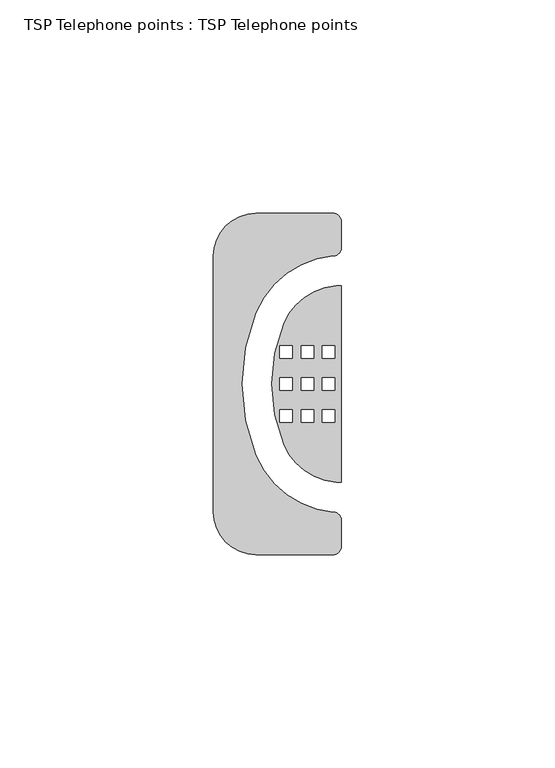
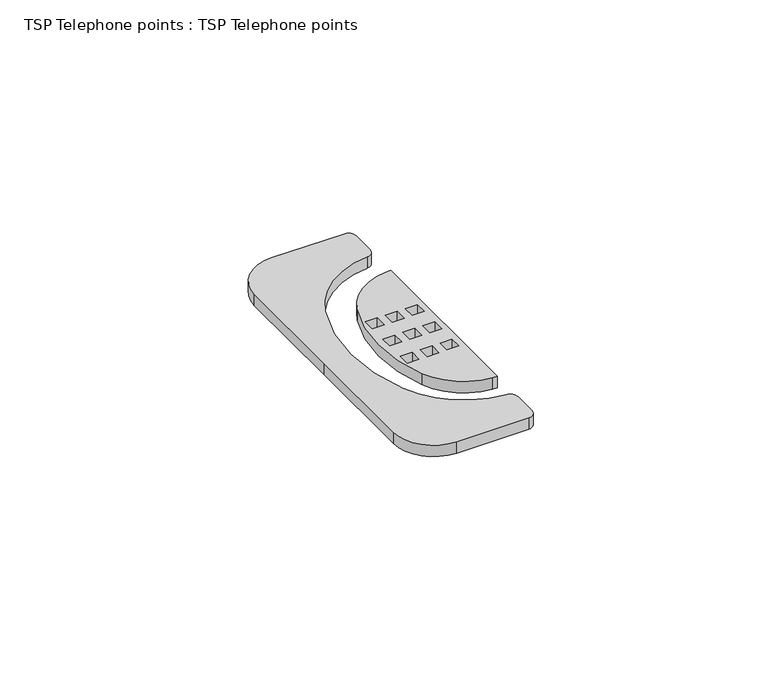
"""IFC4 building model written with IfcOpenShell, lengths in millimetres: proxy geometry, TSP Telephone points : TSP Telephone points."""

from ifc_helpers import new_model, si_unit, point, frame_2d, origin, origin_with_axes, place, context, project, spatial, polyline, circle_curve, trimmed, segment, composite_curve, outline, extrude, source, transform, mapped, element, save


def tsp_telephone_points_tsp_telephone_points_97399d21(model_context):
    return source(origin(), model_context, "Body", "SweptSolid", [
        extrude(outline(composite_curve([segment(polyline([(0.0, 38.0), (0.0, 32.0)]), True, "CONTINUOUS"), segment(trimmed(circle_curve(frame_2d((-2.0, 32.0)), 2.0), [point((0.0, 32.0))], [point((-1.8374907, 30.0066133))], False, "CARTESIAN"), True, "CONTINUOUS"), segment(trimmed(circle_curve(frame_2d((0.0, 8.4180035)), 21.6666667), [point((-1.8374907, 30.0066133))], [point((-20.0, 16.7513368))], True, "CARTESIAN"), True, "CONTINUOUS"), segment(trimmed(circle_curve(frame_2d((20.2032083, 0.0)), 43.5534757), [point((-20.0, 16.7513368))], [point((-20.0, -16.7513368))], True, "CARTESIAN"), True, "CONTINUOUS"), segment(trimmed(circle_curve(frame_2d((0.0, -8.4180035)), 21.6666667), [point((-20.0, -16.7513368))], [point((-1.8374907, -30.0066133))], True, "CARTESIAN"), True, "CONTINUOUS"), segment(trimmed(circle_curve(frame_2d((-2.0, -32.0)), 2.0), [point((-1.8374907, -30.0066133))], [point((0.0, -32.0))], False, "CARTESIAN"), True, "CONTINUOUS"), segment(polyline([(0.0, -32.0), (0.0, -38.0)]), True, "CONTINUOUS"), segment(trimmed(circle_curve(frame_2d((-2.0, -38.0)), 2.0), [point((0.0, -38.0))], [point((-2.0, -40.0))], False, "CARTESIAN"), True, "CONTINUOUS"), segment(polyline([(-2.0, -40.0), (-20.0, -40.0)]), True, "CONTINUOUS"), segment(trimmed(circle_curve(frame_2d((-20.0, -30.0)), 10.0), [point((-20.0, -40.0))], [point((-30.0, -30.0))], False, "CARTESIAN"), True, "CONTINUOUS"), segment(polyline([(-30.0, -30.0), (-30.0, 0.0), (-30.0, 30.0)]), True, "CONTINUOUS"), segment(trimmed(circle_curve(frame_2d((-20.0, 30.0)), 10.0), [point((-30.0, 30.0))], [point((-20.0, 40.0))], False, "CARTESIAN"), True, "CONTINUOUS"), segment(polyline([(-20.0, 40.0), (-2.0, 40.0)]), True, "CONTINUOUS"), segment(trimmed(circle_curve(frame_2d((-2.0, 38.0)), 2.0), [point((-2.0, 40.0))], [point((0.0, 38.0))], False, "CARTESIAN"), True, "CONTINUOUS")], self_intersect=False)), origin_with_axes(), (0.0, 0.0, 1.0), 3.0),
        extrude(outline(composite_curve([segment(trimmed(circle_curve(frame_2d((20.2032083, 0.0)), 36.5534757), [point((-13.5384615, -14.0590291))], [point((-13.5384615, 14.0590291))], False, "CARTESIAN"), True, "CONTINUOUS"), segment(trimmed(circle_curve(frame_2d((0.0, 8.4180035)), 14.6666667), [point((-13.5384615, 14.0590291))], [point((-1.2438398, 23.0318316))], False, "CARTESIAN"), True, "CONTINUOUS"), segment(polyline([(-1.2438398, 23.0318316), (0.0, 23.0318316), (0.0, -23.0318316), (-1.2438398, -23.0318316)]), True, "CONTINUOUS"), segment(trimmed(circle_curve(frame_2d((0.0, -8.4180035)), 14.6666667), [point((-1.2438398, -23.0318316))], [point((-13.5384615, -14.0590291))], False, "CARTESIAN"), True, "CONTINUOUS")], self_intersect=False), holes=[polyline([(-6.4751337, 9.0), (-9.4524255, 9.0), (-9.4524255, 6.0), (-6.4751337, 6.0), (-6.4751337, 9.0)]), polyline([(-11.4751337, 9.0), (-14.4524255, 9.0), (-14.4524255, 6.0), (-11.4751337, 6.0), (-11.4751337, 9.0)]), polyline([(-4.4751337, 9.0), (-4.4751337, 6.0), (-1.4978419, 6.0), (-1.4978419, 9.0), (-4.4751337, 9.0)]), polyline([(-6.4751337, -9.0), (-6.4751337, -6.0), (-9.4524255, -6.0), (-9.4524255, -9.0), (-6.4751337, -9.0)]), polyline([(-11.4751337, -9.0), (-11.4751337, -6.0), (-14.4524255, -6.0), (-14.4524255, -9.0), (-11.4751337, -9.0)]), polyline([(-4.4751337, -9.0), (-1.4978419, -9.0), (-1.4978419, -6.0), (-4.4751337, -6.0), (-4.4751337, -9.0)]), polyline([(-6.4751337, -1.5), (-6.4751337, 1.5), (-9.4524255, 1.5), (-9.4524255, -1.5), (-6.4751337, -1.5)]), polyline([(-11.4751337, -1.5), (-11.4751337, 1.5), (-14.4524255, 1.5), (-14.4524255, -1.5), (-11.4751337, -1.5)]), polyline([(-4.4751337, -1.5), (-1.4978419, -1.5), (-1.4978419, 1.5), (-4.4751337, 1.5), (-4.4751337, -1.5)])]), origin_with_axes(), (0.0, 0.0, 1.0), 3.0),
    ])


if __name__ == "__main__":
    model = new_model("IFC4")
    model_context = context("Model", 3, world=origin())
    ifc_project = project(units=[si_unit("LENGTHUNIT", "METRE", prefix="MILLI")], contexts=[model_context])
    site = spatial("IfcSite", under=ifc_project)
    building = spatial("IfcBuilding", under=site)
    placement = place(None, origin())
    tsp_telephone_points_tsp_telephone_points_shape = tsp_telephone_points_tsp_telephone_points_97399d21(model_context)
    element("IfcBuildingElementProxy", 1, Name="TSP Telephone points : TSP Telephone points", ObjectType="TSP Telephone points : TSP Telephone points", at=placement, inside=building, context=model_context, shape_type="MappedRepresentation", body=[
        mapped(tsp_telephone_points_tsp_telephone_points_shape, transform((0.0, 0.0, 0.0), x_axis=(1.0, 0.0, 0.0), y_axis=(0.0, 1.0, 0.0), z_axis=(0.0, 0.0, 1.0))),
    ])
    save(model, "model.ifc")

# Revit data of these elements
# Type "TSP Telephone points : TSP Telephone points"
#   Model = "TSP_ELECTELP"
#   Default Elevation = 0
# Element 1 (IfcBuildingElementProxy, "TSP Telephone points : TSP Telephone points")
#   Materials on its faces: "Cellulose Fill"
# Materials
#   "Cellulose Fill": class "Generic", colour RGB 0 0 0, transparency 0, Description = "Cellulose loose fill", Cost = 0
